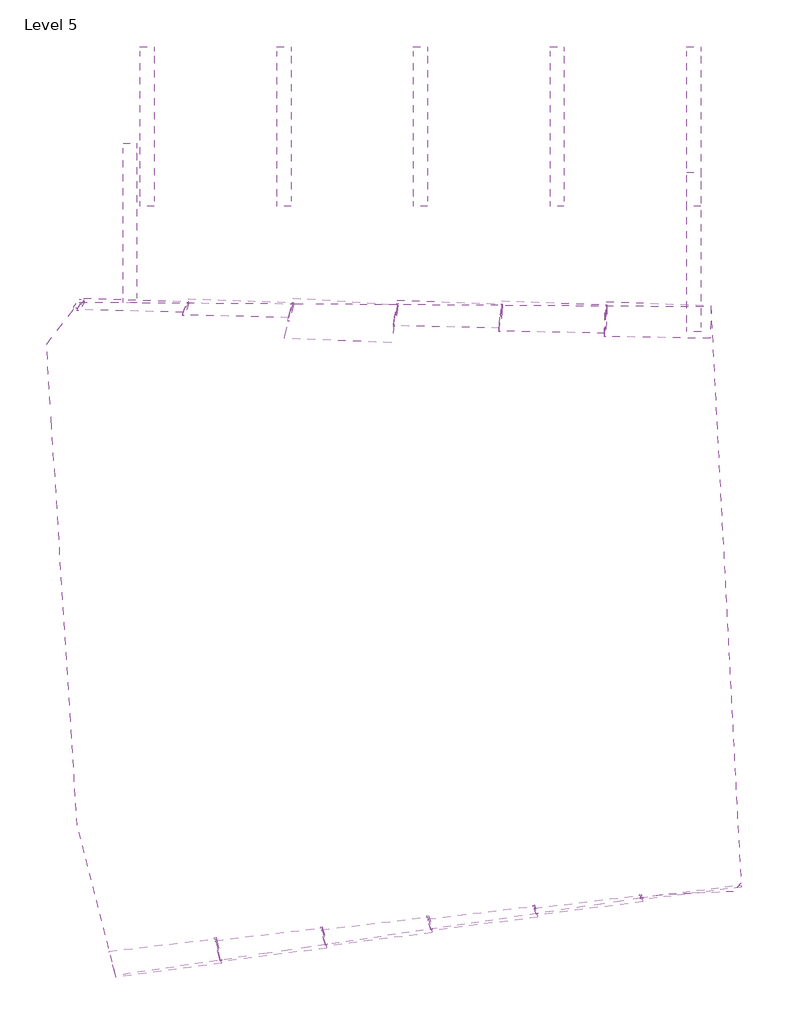
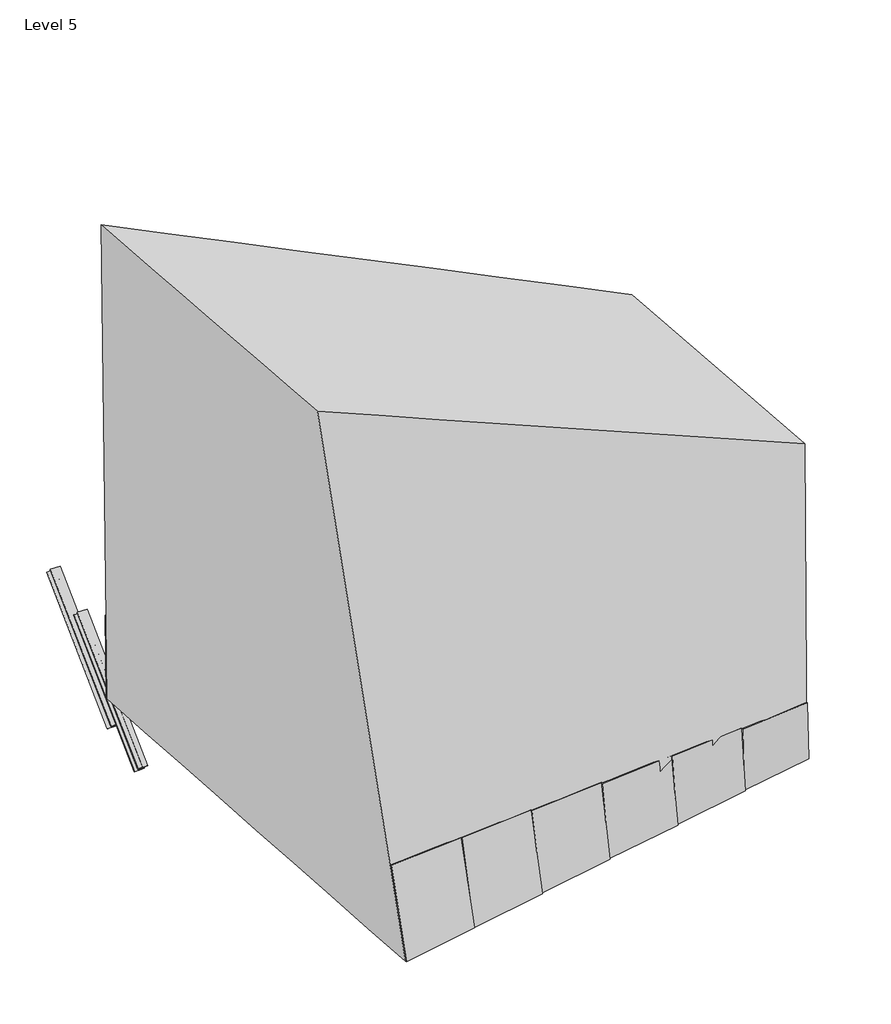
# One storey: 13 plates, 11 members, 7 columns, 1 proxy.
"""IFC4 building model written with IfcOpenShell, lengths in millimetres."""

import ifcopenshell
import ifcopenshell.guid

model = None  # the IFC model being written
_history = None  # IfcOwnerHistory: only IFC2X3 demands one
_inside = {}  # id of a spatial element -> (the spatial element, [elements in it])
_under = {}  # id of a project, library or spatial element -> (it, [spatial elements below it])
_declared = {}  # id of a project -> (the project, [libraries it declares])
_typed = {}  # id of a type object -> (the type object, [elements of that type])
_made_of = {}  # id of a material, layer set ... -> (it, [elements and type objects made of it])


def new_model(schema):
    """Start an empty IFC model of exactly this schema.

    Asked for "IFC4X3", IfcOpenShell would pick the latest addendum, in which some entities
    have other attributes; the version numbers below select the first issue.
    IFC2X3 requires an IfcOwnerHistory on every rooted entity: one is made here for all.
    """
    global model, _history
    if schema == "IFC4X3":
        model = ifcopenshell.file(schema_version=(4, 3, 0, 0))
    else:
        model = ifcopenshell.file(schema=schema)
    _inside.clear()
    _under.clear()
    _declared.clear()
    _typed.clear()
    _made_of.clear()
    _history = None
    if model.schema == "IFC2X3":
        org = make("IfcOrganization", Name="unknown")
        user = make(
            "IfcPersonAndOrganization",
            ThePerson=make("IfcPerson", FamilyName="unknown"),
            TheOrganization=org,
        )
        app = make(
            "IfcApplication",
            ApplicationDeveloper=org,
            Version="unknown",
            ApplicationFullName="unknown",
            ApplicationIdentifier="unknown",
        )
        _history = make(
            "IfcOwnerHistory",
            OwningUser=user,
            OwningApplication=app,
            ChangeAction="ADDED",
            CreationDate=0,
        )
    return model


def make(cls, **values):
    """One entity of the class cls with the attributes given. An attribute that is None is left unset."""
    return model.create_entity(
        cls, **{name: value for name, value in values.items() if value is not None}
    )


def rooted(cls, **values):
    """An entity with a GlobalId (a new one), such as an element, a storey or a relation."""
    return make(cls, GlobalId=ifcopenshell.guid.new(), OwnerHistory=_history, **values)


def si_unit(unit_type, name, prefix=None):
    """IfcSIUnit, for example si_unit("LENGTHUNIT", "METRE", prefix="MILLI")."""
    return make("IfcSIUnit", UnitType=unit_type, Prefix=prefix, Name=name)


def assignment(units):
    """IfcUnitAssignment: the units of a project."""
    return None if units is None else make("IfcUnitAssignment", Units=units)


def point(xyz):
    """IfcCartesianPoint."""
    return None if xyz is None else make("IfcCartesianPoint", Coordinates=xyz)


def direction(xyz):
    """IfcDirection."""
    return None if xyz is None else make("IfcDirection", DirectionRatios=xyz)


def frame(location, z_axis=None, x_axis=None):
    """IfcAxis2Placement3D, a coordinate frame: its origin and axes. An axis left out is left unset."""
    return make(
        "IfcAxis2Placement3D",
        Location=point(location),
        Axis=direction(z_axis),
        RefDirection=direction(x_axis),
    )


def frame_2d(location, x_axis=None):
    """IfcAxis2Placement2D, a coordinate frame in the plane: its origin and x axis."""
    return make(
        "IfcAxis2Placement2D", Location=point(location), RefDirection=direction(x_axis)
    )


def origin():
    """The frame at (0, 0, 0) with its axes left unset."""
    return frame((0.0, 0.0, 0.0))


def place(relative_to, where):
    """IfcLocalPlacement: puts the frame where relative to a parent placement (None: the world)."""
    return make(
        "IfcLocalPlacement", PlacementRelTo=relative_to, RelativePlacement=where
    )


def context(
    kind, dimensions, precision=None, world=None, true_north=None, identifier=None
):
    """IfcGeometricRepresentationContext, for example the 3D "Model" context."""
    return make(
        "IfcGeometricRepresentationContext",
        ContextIdentifier=identifier,
        ContextType=kind,
        CoordinateSpaceDimension=dimensions,
        Precision=precision,
        WorldCoordinateSystem=world,
        TrueNorth=true_north,
    )


def project(units=None, contexts=None):
    """IfcProject with its units and contexts."""
    return rooted(
        "IfcProject",
        Name="project",
        RepresentationContexts=contexts,
        UnitsInContext=assignment(units),
    )


def spatial(cls, under=None, at=None, **own):
    """A site, building, storey or space (cls), placed at a placement, below another one or the project."""
    s = rooted(cls, ObjectPlacement=at, **own)
    if under is not None:
        _under.setdefault(under.id(), (under, []))[1].append(s)
    return s


def polyline(points):
    """IfcPolyline through the points."""
    return make("IfcPolyline", Points=[point(p) for p in points])


def circle_curve(where, radius):
    """IfcCircle in the frame where."""
    return make("IfcCircle", Position=where, Radius=radius)


def trimmed(basis, trim1, trim2, sense, master):
    """IfcTrimmedCurve: the piece of a basis curve between two trims."""
    return make(
        "IfcTrimmedCurve",
        BasisCurve=basis,
        Trim1=trim1,
        Trim2=trim2,
        SenseAgreement=sense,
        MasterRepresentation=master,
    )


def segment(curve, same_sense, transition):
    """IfcCompositeCurveSegment."""
    return make(
        "IfcCompositeCurveSegment",
        Transition=transition,
        SameSense=same_sense,
        ParentCurve=curve,
    )


def composite_curve(segments, self_intersect=None):
    """IfcCompositeCurve: segments joined end to end."""
    return make("IfcCompositeCurve", Segments=segments, SelfIntersect=self_intersect)


def outline(outer, holes=None, kind="AREA"):
    """IfcArbitraryClosedProfileDef: a profile drawn as a closed curve; with holes, ...WithVoids."""
    if holes is None:
        return make("IfcArbitraryClosedProfileDef", ProfileType=kind, OuterCurve=outer)
    return make(
        "IfcArbitraryProfileDefWithVoids",
        ProfileType=kind,
        OuterCurve=outer,
        InnerCurves=holes,
    )


def extrude(swept, where, along, depth):
    """IfcExtrudedAreaSolid: the profile swept, set in the frame where, extruded along a direction by depth."""
    return make(
        "IfcExtrudedAreaSolid",
        SweptArea=swept,
        Position=where,
        ExtrudedDirection=direction(along),
        Depth=depth,
    )


def shape(context_of_items, identifier, shape_type, items):
    """IfcShapeRepresentation: the items that make up one representation, for example the "Body"."""
    return make(
        "IfcShapeRepresentation",
        ContextOfItems=context_of_items,
        RepresentationIdentifier=identifier,
        RepresentationType=shape_type,
        Items=items,
    )


def source(mapping_origin, context_of_items, identifier, shape_type, items):
    """IfcRepresentationMap: a shape defined once, which mapped items show again and again."""
    return make(
        "IfcRepresentationMap",
        MappingOrigin=mapping_origin,
        MappedRepresentation=shape(context_of_items, identifier, shape_type, items),
    )


def transform(
    local_origin,
    x_axis=None,
    y_axis=None,
    z_axis=None,
    scale=None,
    scale2=None,
    scale3=None,
    uniform=True,
):
    """IfcCartesianTransformationOperator3D, or its non-uniform kind. x_axis, y_axis, z_axis: its Axis1, 2, 3."""
    if uniform:
        return make(
            "IfcCartesianTransformationOperator3D",
            Axis1=direction(x_axis),
            Axis2=direction(y_axis),
            LocalOrigin=point(local_origin),
            Scale=scale,
            Axis3=direction(z_axis),
        )
    return make(
        "IfcCartesianTransformationOperator3DnonUniform",
        Axis1=direction(x_axis),
        Axis2=direction(y_axis),
        LocalOrigin=point(local_origin),
        Scale=scale,
        Axis3=direction(z_axis),
        Scale2=scale2,
        Scale3=scale3,
    )


def mapped(mapping_source, mapping_target):
    """IfcMappedItem: shows the shape of a source again, moved by a transform."""
    return make(
        "IfcMappedItem", MappingSource=mapping_source, MappingTarget=mapping_target
    )


def made_of(thing, what):
    """Note that an element or type object is made of a material, layer set ...; save() writes the relation."""
    if what is not None:
        _made_of.setdefault(what.id(), (what, []))[1].append(thing)
    return thing


def element(
    cls,
    number,
    at=None,
    inside=None,
    cuts=None,
    type_object=None,
    material=None,
    context=None,
    identifier="Body",
    shape_type=None,
    held_by="IfcProductDefinitionShape",
    body=None,
    shapes=None,
    **own,
):
    """One element of the class cls, such as IfcWall. Its Tag is "e" and its number.

    at: its placement. inside: the storey or other place that contains it. cuts: it is an
    opening in that element (IfcRelVoidsElement). A single representation is given by context,
    identifier, shape_type and body (its items); several are given by shapes. held_by: the class
    of the entity that holds the representations. save() writes the other relations.
    """
    e = rooted(cls, Tag="e%d" % number, ObjectPlacement=at, **own)
    if body is not None:
        shapes = [shape(context, identifier, shape_type, body)]
    if shapes is not None:
        e.Representation = make(held_by, Representations=shapes)
    if inside is not None:
        _inside.setdefault(inside.id(), (inside, []))[1].append(e)
    if cuts is not None:
        rooted(
            "IfcRelVoidsElement", RelatingBuildingElement=cuts, RelatedOpeningElement=e
        )
    if type_object is not None:
        _typed.setdefault(type_object.id(), (type_object, []))[1].append(e)
    return made_of(e, material)


def aggregate(whole, parts):
    """IfcRelAggregates: a whole, such as a stair, and the parts it consists of."""
    return rooted("IfcRelAggregates", RelatingObject=whole, RelatedObjects=parts)


def save(model, path):
    """Write the relations noted so far, then the file.

    IfcRelAggregates (storeys below a building ...), IfcRelContainedInSpatialStructure (elements
    in a storey), IfcRelDefinesByType, IfcRelAssociatesMaterial and IfcRelDeclares: one each for
    every whole, place, type object, material and project.
    """
    for whole, parts in _under.values():
        aggregate(whole, parts)
    for where, things in _inside.values():
        rooted(
            "IfcRelContainedInSpatialStructure",
            RelatedElements=things,
            RelatingStructure=where,
        )
    for kind, things in _typed.values():
        rooted("IfcRelDefinesByType", RelatedObjects=things, RelatingType=kind)
    for what, things in _made_of.values():
        rooted("IfcRelAssociatesMaterial", RelatedObjects=things, RelatingMaterial=what)
    for by, libraries in _declared.values():
        rooted("IfcRelDeclares", RelatingContext=by, RelatedDefinitions=libraries)
    model.write(path)


def spline_surface(u_degree, v_degree, points, u_multiplicities, v_multiplicities, u_knots, v_knots, weights=None):
    """IfcBSplineSurfaceWithKnots; with weights, IfcRationalBSplineSurfaceWithKnots. points: one row for each step in u."""
    own = dict(
        UDegree=u_degree,
        VDegree=v_degree,
        ControlPointsList=[[point(p) for p in row] for row in points],
        SurfaceForm="UNSPECIFIED",
        UClosed=False,
        VClosed=False,
        SelfIntersect=False,
        UMultiplicities=u_multiplicities,
        VMultiplicities=v_multiplicities,
        UKnots=u_knots,
        VKnots=v_knots,
        KnotSpec="UNSPECIFIED",
    )
    if weights is None:
        return make("IfcBSplineSurfaceWithKnots", **own)
    return make("IfcRationalBSplineSurfaceWithKnots", WeightsData=weights, **own)


def advanced_brep(points, edges, surfaces, faces):
    """IfcAdvancedBrep: a solid bounded by faces that lie on surfaces and meet in shared edges.

    An edge is (start, end): straight between two places in points (the first is 0);
    or (start, end, curve); or (start, end, curve, False) where it runs against its curve.
    A face is (place in surfaces, loops), or (place, loops, False) where it looks against
    its surface's normal. A loop lists edges by number (the first is 1), with a minus sign
    where the edge is run from its end to its start. The first loop is the outer one.
    """
    corners = [point(p) for p in points]
    vertices = [make("IfcVertexPoint", VertexGeometry=c) for c in corners]
    made = []
    for start, end, *more in edges:
        made.append(
            make(
                "IfcEdgeCurve",
                EdgeStart=vertices[start],
                EdgeEnd=vertices[end],
                EdgeGeometry=more[0] if more else make("IfcPolyline", Points=[corners[start], corners[end]]),
                SameSense=more[1] if len(more) > 1 else True,
            )
        )
    hull = []
    for where, loops, *sense in faces:
        bounds = []
        for j, loop in enumerate(loops):
            ring = [make("IfcOrientedEdge", EdgeElement=made[abs(k) - 1], Orientation=k > 0) for k in loop]
            bounds.append(
                make(
                    "IfcFaceOuterBound" if j == 0 else "IfcFaceBound",
                    Bound=make("IfcEdgeLoop", EdgeList=ring),
                    Orientation=True,
                )
            )
        hull.append(make("IfcAdvancedFace", Bounds=bounds, FaceSurface=surfaces[where], SameSense=sense[0] if sense else True))
    return make("IfcAdvancedBrep", Outer=make("IfcClosedShell", CfsFaces=hull))


def rectangular_mullion_30mm_square_281b7b6d(model_context):
    return source(origin(), model_context, "Body", "SweptSolid", [
        extrude(outline(polyline([(15.0, 15.0), (15.0, -15.0), (-15.0, -15.0), (-15.0, 15.0), (15.0, 15.0)])), frame((0.0, 0.0, -1763.4174675), z_axis=(0.0, 0.0, 1.0), x_axis=(1.0, 0.0, 0.0)), (0.0, 0.0, 1.0), 1763.4174675),
    ])


def rectangular_mullion_30mm_square_c8a39bf0(model_context):
    return source(origin(), model_context, "Body", "SweptSolid", [
        extrude(outline(polyline([(15.0, 15.0), (15.0, -15.0), (-15.0, -15.0), (-15.0, 15.0), (15.0, 15.0)])), frame((0.0, 0.0, -1876.7376356), z_axis=(0.0, 0.0, 1.0), x_axis=(1.0, 0.0, 0.0)), (0.0, 0.0, 1.0), 1876.7376356),
    ])


def rectangular_mullion_30mm_square_b082ce79(model_context):
    return source(origin(), model_context, "Body", "SweptSolid", [
        extrude(outline(polyline([(15.0, 15.0), (15.0, -15.0), (-15.0, -15.0), (-15.0, 15.0), (15.0, 15.0)])), frame((0.0, 0.0, -1997.4407133), z_axis=(0.0, 0.0, 1.0), x_axis=(1.0, 0.0, 0.0)), (0.0, 0.0, 1.0), 1997.4407133),
    ])


def rectangular_mullion_30mm_square_a1c2493b(model_context):
    return source(origin(), model_context, "Body", "SweptSolid", [
        extrude(outline(polyline([(15.0, 15.0), (15.0, -15.0), (-15.0, -15.0), (-15.0, 15.0), (15.0, 15.0)])), frame((0.0, 0.0, -2124.2685603), z_axis=(0.0, 0.0, 1.0), x_axis=(1.0, 0.0, 0.0)), (0.0, 0.0, 1.0), 2124.2685603),
    ])


def rectangular_mullion_30mm_square_b3fc8657(model_context):
    return source(origin(), model_context, "Body", "SweptSolid", [
        extrude(outline(polyline([(15.0, 15.0), (15.0, -15.0), (-15.0, -15.0), (-15.0, 15.0), (15.0, 15.0)])), frame((0.0, 0.0, -2256.188532), z_axis=(0.0, 0.0, 1.0), x_axis=(1.0, 0.0, 0.0)), (0.0, 0.0, 1.0), 2256.188532),
    ])


def rectangular_mullion_30mm_square_3a89077b(model_context):
    return source(origin(), model_context, "Body", "SweptSolid", [
        extrude(outline(polyline([(15.0, 15.0), (15.0, -15.0), (-15.0, -15.0), (-15.0, 15.0), (15.0, 15.0)])), frame((0.0, 0.0, -2392.3584034), z_axis=(0.0, 0.0, 1.0), x_axis=(1.0, 0.0, 0.0)), (0.0, 0.0, 1.0), 2392.3584034),
    ])


def rectangular_mullion_30mm_square_25ecd6b2(model_context):
    return source(origin(), model_context, "Body", "SweptSolid", [
        extrude(outline(polyline([(15.0, 15.0), (15.0, -15.0), (-15.0, -15.0), (-15.0, 15.0), (15.0, 15.0)])), frame((0.0, 0.0, -2311.5857878), z_axis=(0.0, 0.0, 1.0), x_axis=(1.0, 0.0, 0.0)), (0.0, 0.0, 1.0), 2311.5857878),
    ])


def rectangular_mullion_30mm_square_fecaf73a(model_context):
    return source(origin(), model_context, "Body", "SweptSolid", [
        extrude(outline(polyline([(15.0, 15.0), (15.0, -15.0), (-15.0, -15.0), (-15.0, 15.0), (15.0, 15.0)])), frame((0.0, 0.0, -2152.3545613), z_axis=(0.0, 0.0, 1.0), x_axis=(1.0, 0.0, 0.0)), (0.0, 0.0, 1.0), 2152.3545613),
    ])


def rectangular_mullion_30mm_square_a7719491(model_context):
    return source(origin(), model_context, "Body", "SweptSolid", [
        extrude(outline(polyline([(15.0, 15.0), (15.0, -15.0), (-15.0, -15.0), (-15.0, 15.0), (15.0, 15.0)])), frame((0.0, 0.0, -1995.0714456), z_axis=(0.0, 0.0, 1.0), x_axis=(1.0, 0.0, 0.0)), (0.0, 0.0, 1.0), 1995.0714456),
    ])


def rectangular_mullion_30mm_square_8e68c213(model_context):
    return source(origin(), model_context, "Body", "SweptSolid", [
        extrude(outline(polyline([(15.0, 15.0), (15.0, -15.0), (-15.0, -15.0), (-15.0, 15.0), (15.0, 15.0)])), frame((0.0, 0.0, -1840.2360175), z_axis=(0.0, 0.0, 1.0), x_axis=(1.0, 0.0, 0.0)), (0.0, 0.0, 1.0), 1840.2360175),
    ])


def rectangular_mullion_30mm_square_54935cf5(model_context):
    return source(origin(), model_context, "Body", "SweptSolid", [
        extrude(outline(polyline([(15.0, 15.0), (15.0, -15.0), (-15.0, -15.0), (-15.0, 15.0), (15.0, 15.0)])), frame((0.0, 0.0, -1688.5217616), z_axis=(0.0, 0.0, 1.0), x_axis=(1.0, 0.0, 0.0)), (0.0, 0.0, 1.0), 1688.5217616),
    ])


def system_panel_glazed_61bd3bb4(model_context):
    return source(origin(), model_context, "Body", "SweptSolid", [
        extrude(outline(polyline([(0.0, -918.1552821), (0.0, 996.0695243), (1761.0937074, 931.9438881), (1655.9323013, -996.0695243), (0.0, -918.1552821)])), frame((0.0, -49.5, 0.0), z_axis=(0.0, 1.0, 0.0), x_axis=(0.0, 0.0, 1.0)), (0.0, 0.0, 1.0), 25.0),
    ])


def system_panel_glazed_ae3b4f36(model_context):
    return source(origin(), model_context, "Body", "SweptSolid", [
        extrude(outline(polyline([(0.0, -923.1075404), (0.0, 991.2413385), (1874.9756018, 936.3989323), (1761.0780772, -991.2413385), (0.0, -923.1075404)])), frame((0.0, -49.5, 0.0), z_axis=(0.0, 1.0, 0.0), x_axis=(0.0, 0.0, 1.0)), (0.0, 0.0, 1.0), 25.0),
    ])


def system_panel_glazed_7d8b04ef(model_context):
    return source(origin(), model_context, "Body", "SweptSolid", [
        extrude(outline(polyline([(0.0, -937.8383573), (0.0, 976.8018413), (2255.477521, 949.9625368), (2123.3255208, -976.8018413), (0.0, -937.8383573)])), frame((0.0, -49.5, 0.0), z_axis=(0.0, 1.0, 0.0), x_axis=(0.0, 0.0, 1.0)), (0.0, 0.0, 1.0), 25.0),
    ])


def system_panel_glazed_3b9d15b0(model_context):
    return source(origin(), model_context, "Body", "SweptSolid", [
        extrude(outline(polyline([(0.0, -942.7108166), (0.0, 972.0020553), (2391.8329241, 954.5438482), (2255.5087034, -972.0020553), (0.0, -942.7108166)])), frame((0.0, -49.5, 0.0), z_axis=(0.0, 1.0, 0.0), x_axis=(0.0, 0.0, 1.0)), (0.0, 0.0, 1.0), 25.0),
    ])


def system_panel_glazed_4dd55457(model_context):
    return source(origin(), model_context, "Body", "SweptSolid", [
        extrude(outline(polyline([(0.0, -30.1852095), (0.0, 48.8417218), (2397.9897252, 30.6680018), (2392.2849165, -48.8417218), (0.0, -30.1852095)])), frame((0.0, -49.5, 0.0), z_axis=(0.0, 1.0, 0.0), x_axis=(0.0, 0.0, 1.0)), (0.0, 0.0, 1.0), 25.0),
    ])


def system_panel_glazed_c41e03b4(model_context):
    return source(origin(), model_context, "Body", "SweptSolid", [
        extrude(outline(polyline([(0.0, -1008.7560992), (0.0, 941.2557286), (2310.4175162, 1008.7560992), (2471.2238346, -938.6456704), (0.0, -1008.7560992)])), frame((0.0, -49.5, 0.0), z_axis=(0.0, 1.0, 0.0), x_axis=(0.0, 0.0, 1.0)), (0.0, 0.0, 1.0), 25.0),
    ])


def system_panel_glazed_15b89219(model_context):
    return source(origin(), model_context, "Body", "SweptSolid", [
        extrude(outline(polyline([(0.0, -1007.0351176), (0.0, 942.9445704), (2151.1749822, 1007.0351176), (2310.4173325, -940.4629834), (0.0, -1007.0351176)])), frame((0.0, -49.5, 0.0), z_axis=(0.0, 1.0, 0.0), x_axis=(0.0, 0.0, 1.0)), (0.0, 0.0, 1.0), 25.0),
    ])


def system_panel_glazed_cfa6e621(model_context):
    return source(origin(), model_context, "Body", "SweptSolid", [
        extrude(outline(polyline([(0.0, -1005.3178204), (0.0, 944.6224941), (1993.8665555, 1005.3178204), (2151.1709359, -942.2983527), (0.0, -1005.3178204)])), frame((0.0, -49.5, 0.0), z_axis=(0.0, 1.0, 0.0), x_axis=(0.0, 0.0, 1.0)), (0.0, 0.0, 1.0), 25.0),
    ])


def system_panel_glazed_fa6ac5bb(model_context):
    return source(origin(), model_context, "Body", "SweptSolid", [
        extrude(outline(polyline([(0.0, -1003.6052901), (0.0, 946.2862543), (1838.9863035, 1003.6052901), (1993.8564357, -944.1571371), (0.0, -1003.6052901)])), frame((0.0, -49.5, 0.0), z_axis=(0.0, 1.0, 0.0), x_axis=(0.0, 0.0, 1.0)), (0.0, 0.0, 1.0), 25.0),
    ])


def system_panel_glazed_53210cc6(model_context):
    return source(origin(), model_context, "Body", "SweptSolid", [
        extrude(outline(polyline([(0.0, -1001.8989904), (0.0, 947.931492), (1687.1996383, 1001.8989904), (1838.9666874, -946.0465604), (0.0, -1001.8989904)])), frame((0.0, -49.5, 0.0), z_axis=(0.0, 1.0, 0.0), x_axis=(0.0, 0.0, 1.0)), (0.0, 0.0, 1.0), 25.0),
    ])


def system_panel_glazed_08f6996d(model_context):
    return source(origin(), model_context, "Body", "SweptSolid", [
        extrude(outline(polyline([(0.0, -938.7563704), (0.0, 887.9536467), (1548.6739711, 938.7563704), (1687.2330704, -886.4668133), (0.0, -938.7563704)])), frame((0.0, -49.5, 0.0), z_axis=(0.0, 1.0, 0.0), x_axis=(0.0, 0.0, 1.0)), (0.0, 0.0, 1.0), 25.0),
    ])


def system_panel_glazed_6e61295c(model_context):
    return source(origin(), model_context, "Body", "SweptSolid", [
        extrude(outline(polyline([(0.0, -906.0305588), (0.0, 1006.3483292), (2123.3277595, 971.552521), (4246.6555191, 936.7567127), (3992.2264945, -1006.3483292), (1996.1132472, -956.189444), (0.0, -906.0305588)])), frame((0.0, -49.5, 0.0), z_axis=(0.0, 1.0, 0.0), x_axis=(0.0, 0.0, 1.0)), (0.0, 0.0, 1.0), 25.0),
    ])


def system_panel_glazed_31f0a782(model_context):
    return source(origin(), model_context, "Body", "SweptSolid", [
        extrude(outline(polyline([(0.0, -928.0385226), (0.0, 986.4208083), (1996.1252593, 940.8873527), (1874.9814945, -986.4208083), (0.0, -928.0385226)])), frame((0.0, -49.5, 0.0), z_axis=(0.0, 1.0, 0.0), x_axis=(0.0, 0.0, 1.0)), (0.0, 0.0, 1.0), 25.0),
    ])


model = new_model("IFC4")

# Units and contexts
model_context = context("Model", 3, world=origin())
ifc_project = project(units=[si_unit("LENGTHUNIT", "METRE", prefix="MILLI")], contexts=[model_context])

# Site, building, storey
site = spatial("IfcSite", under=ifc_project)
building = spatial("IfcBuilding", under=site)
storey = spatial("IfcBuildingStorey", under=building, Name="Level 5", Elevation=-5000.0)

# Proxy
placement = place(None, origin())
element("IfcBuildingElementProxy", 1, Name="volumen2 : volumen2", ObjectType="volumen2 : volumen2", at=placement, inside=storey, context=model_context, shape_type="AdvancedBrep", body=[
    advanced_brep(
    [(-4919.3716289, 29199.3093249, 0.0), (-5472.2265132, 39751.3413148, 0.0), (-5508.4633275, 36083.0409484, 8786.8733417), (-5062.165814, 29050.9821784, 8786.8733417), (-17027.8343957, 39830.0880172, -587.2378435), (-17626.1101206, 39059.1200592, 13141.9598572), (-16359.3479239, 27514.3891838, -587.2378435), (-17064.1810196, 30263.3944457, 13141.9598572)],
    [
        (0, 1),
        (1, 2),
        (2, 3),
        (3, 0),
        (1, 4),
        (4, 5),
        (5, 2),
        (4, 6),
        (6, 7),
        (7, 5),
        (6, 0),
        (3, 7),
    ],
    [
        spline_surface(1, 1, [[(-4919.3716289, 29199.3093249, 0.0), (-5062.165814, 29050.9821784, 8786.8733417)], [(-5472.2265132, 39751.3413148, 0.0), (-5508.4633275, 36083.0409484, 8786.8733417)]], [2, 2], [2, 2], [0.0, 1.0], [0.0, 1.0]),
        spline_surface(1, 1, [[(-5472.2265132, 39751.3413148, 0.0), (-5508.4633275, 36083.0409484, 8786.8733417)], [(-17027.8343957, 39830.0880172, -587.2378435), (-17626.1101206, 39059.1200592, 13141.9598572)]], [2, 2], [2, 2], [0.0, 1.0], [0.0, 1.0]),
        spline_surface(1, 1, [[(-17027.8343957, 39830.0880172, -587.2378435), (-17626.1101206, 39059.1200592, 13141.9598572)], [(-16359.3479239, 27514.3891838, -587.2378435), (-17064.1810196, 30263.3944457, 13141.9598572)]], [2, 2], [2, 2], [0.0, 1.0], [0.0, 1.0]),
        spline_surface(1, 1, [[(-16359.3479239, 27514.3891838, -587.2378435), (-17064.1810196, 30263.3944457, 13141.9598572)], [(-4919.3716289, 29199.3093249, 0.0), (-5062.165814, 29050.9821784, 8786.8733417)]], [2, 2], [2, 2], [0.0, 1.0], [0.0, 1.0]),
        spline_surface(1, 1, [[(-17064.1810196, 30263.3944457, 13141.9598572), (-17626.1101206, 39059.1200592, 13141.9598572)], [(-5062.165814, 29050.9821784, 8786.8733417), (-5508.4633275, 36083.0409484, 8786.8733417)]], [2, 2], [2, 2], [0.0, 1.0], [0.0, 1.0]),
        spline_surface(1, 1, [[(-16359.3479239, 27514.3891838, -587.2378435), (-4919.3716289, 29199.3093249, 0.0)], [(-17027.8343957, 39830.0880172, -587.2378435), (-5472.2265132, 39751.3413148, 0.0)]], [2, 2], [2, 2], [0.0, 1.0], [0.0, 1.0]),
    ],
    [
        (0, [[1, 2, 3, 4]]),
        (1, [[5, 6, 7, -2]]),
        (2, [[8, 9, 10, -6]]),
        (3, [[11, -4, 12, -9]]),
        (4, [[-10, -12, -3, -7]]),
        (5, [[-11, -8, -5, -1]]),
    ],
),
])

# Columns
element("IfcColumn", 2, ObjectType="M_W Shapes-Column : W250X73", at=placement, inside=storey, context=model_context, shape_type="SweptSolid", body=[
    extrude(outline(composite_curve([segment(polyline([(254.0, 0.0), (254.0, -14.2), (144.02, -14.2)]), True, "CONTINUOUS"), segment(trimmed(circle_curve(frame_2d((144.02, -26.9)), 12.7), [point((144.02, -14.2))], [point((131.32, -26.9))], True, "CARTESIAN"), True, "CONTINUOUS"), segment(polyline([(131.32, -26.9), (131.32, -227.1)]), True, "CONTINUOUS"), segment(trimmed(circle_curve(frame_2d((144.02, -227.1)), 12.7), [point((131.32, -227.1))], [point((144.02, -239.8))], True, "CARTESIAN"), True, "CONTINUOUS"), segment(polyline([(144.02, -239.8), (254.0, -239.8), (254.0, -254.0), (0.0, -254.0), (0.0, -239.8), (109.98, -239.8)]), True, "CONTINUOUS"), segment(trimmed(circle_curve(frame_2d((109.98, -227.1)), 12.7), [point((109.98, -239.8))], [point((122.68, -227.1))], True, "CARTESIAN"), True, "CONTINUOUS"), segment(polyline([(122.68, -227.1), (122.68, -26.9)]), True, "CONTINUOUS"), segment(trimmed(circle_curve(frame_2d((109.98, -26.9)), 12.7), [point((122.68, -26.9))], [point((109.98, -14.2))], True, "CARTESIAN"), True, "CONTINUOUS"), segment(polyline([(109.98, -14.2), (0.0, -14.2), (0.0, 0.0), (254.0, 0.0)]), True, "CONTINUOUS")], self_intersect=False)), frame((-5654.6382157, 41587.2616115, -2795.3553834), z_axis=(0.0, 0.7184819062976688, 0.6955456493450793), x_axis=(-1.0, 0.0, 0.0)), (0.0, 0.0, 1.0), 3813.3951187),
])
element("IfcColumn", 3, ObjectType="M_W Shapes-Column : W250X73", at=placement, inside=storey, context=model_context, shape_type="SweptSolid", body=[
    extrude(outline(composite_curve([segment(polyline([(254.0, 0.0), (254.0, -14.2), (144.02, -14.2)]), True, "CONTINUOUS"), segment(trimmed(circle_curve(frame_2d((144.02, -26.9)), 12.7), [point((144.02, -14.2))], [point((131.32, -26.9))], True, "CARTESIAN"), True, "CONTINUOUS"), segment(polyline([(131.32, -26.9), (131.32, -227.1)]), True, "CONTINUOUS"), segment(trimmed(circle_curve(frame_2d((144.02, -227.1)), 12.7), [point((131.32, -227.1))], [point((144.02, -239.8))], True, "CARTESIAN"), True, "CONTINUOUS"), segment(polyline([(144.02, -239.8), (254.0, -239.8), (254.0, -254.0), (0.0, -254.0), (0.0, -239.8), (109.98, -239.8)]), True, "CONTINUOUS"), segment(trimmed(circle_curve(frame_2d((109.98, -227.1)), 12.7), [point((109.98, -239.8))], [point((122.68, -227.1))], True, "CARTESIAN"), True, "CONTINUOUS"), segment(polyline([(122.68, -227.1), (122.68, -26.9)]), True, "CONTINUOUS"), segment(trimmed(circle_curve(frame_2d((109.98, -26.9)), 12.7), [point((122.68, -26.9))], [point((109.98, -14.2))], True, "CARTESIAN"), True, "CONTINUOUS"), segment(polyline([(109.98, -14.2), (0.0, -14.2), (0.0, 0.0), (254.0, 0.0)]), True, "CONTINUOUS")], self_intersect=False)), frame((-8154.6382157, 41587.2616115, -2795.3553834), z_axis=(0.0, 0.7184819062976688, 0.6955456493450793), x_axis=(-1.0, 0.0, 0.0)), (0.0, 0.0, 1.0), 3813.3951187),
])
element("IfcColumn", 4, ObjectType="M_W Shapes-Column : W250X73", at=placement, inside=storey, context=model_context, shape_type="SweptSolid", body=[
    extrude(outline(composite_curve([segment(polyline([(254.0, 0.0), (254.0, -14.2), (144.02, -14.2)]), True, "CONTINUOUS"), segment(trimmed(circle_curve(frame_2d((144.02, -26.9)), 12.7), [point((144.02, -14.2))], [point((131.32, -26.9))], True, "CARTESIAN"), True, "CONTINUOUS"), segment(polyline([(131.32, -26.9), (131.32, -227.1)]), True, "CONTINUOUS"), segment(trimmed(circle_curve(frame_2d((144.02, -227.1)), 12.7), [point((131.32, -227.1))], [point((144.02, -239.8))], True, "CARTESIAN"), True, "CONTINUOUS"), segment(polyline([(144.02, -239.8), (254.0, -239.8), (254.0, -254.0), (0.0, -254.0), (0.0, -239.8), (109.98, -239.8)]), True, "CONTINUOUS"), segment(trimmed(circle_curve(frame_2d((109.98, -227.1)), 12.7), [point((109.98, -239.8))], [point((122.68, -227.1))], True, "CARTESIAN"), True, "CONTINUOUS"), segment(polyline([(122.68, -227.1), (122.68, -26.9)]), True, "CONTINUOUS"), segment(trimmed(circle_curve(frame_2d((109.98, -26.9)), 12.7), [point((122.68, -26.9))], [point((109.98, -14.2))], True, "CARTESIAN"), True, "CONTINUOUS"), segment(polyline([(109.98, -14.2), (0.0, -14.2), (0.0, 0.0), (254.0, 0.0)]), True, "CONTINUOUS")], self_intersect=False)), frame((-10654.6382157, 41587.2616115, -2795.3553834), z_axis=(0.0, 0.7184819062976688, 0.6955456493450793), x_axis=(-1.0, 0.0, 0.0)), (0.0, 0.0, 1.0), 3813.3951187),
])
element("IfcColumn", 5, ObjectType="M_W Shapes-Column : W250X73", at=placement, inside=storey, context=model_context, shape_type="SweptSolid", body=[
    extrude(outline(composite_curve([segment(polyline([(254.0, 0.0), (254.0, -14.2), (144.02, -14.2)]), True, "CONTINUOUS"), segment(trimmed(circle_curve(frame_2d((144.02, -26.9)), 12.7), [point((144.02, -14.2))], [point((131.32, -26.9))], True, "CARTESIAN"), True, "CONTINUOUS"), segment(polyline([(131.32, -26.9), (131.32, -227.1)]), True, "CONTINUOUS"), segment(trimmed(circle_curve(frame_2d((144.02, -227.1)), 12.7), [point((131.32, -227.1))], [point((144.02, -239.8))], True, "CARTESIAN"), True, "CONTINUOUS"), segment(polyline([(144.02, -239.8), (254.0, -239.8), (254.0, -254.0), (0.0, -254.0), (0.0, -239.8), (109.98, -239.8)]), True, "CONTINUOUS"), segment(trimmed(circle_curve(frame_2d((109.98, -227.1)), 12.7), [point((109.98, -239.8))], [point((122.68, -227.1))], True, "CARTESIAN"), True, "CONTINUOUS"), segment(polyline([(122.68, -227.1), (122.68, -26.9)]), True, "CONTINUOUS"), segment(trimmed(circle_curve(frame_2d((109.98, -26.9)), 12.7), [point((122.68, -26.9))], [point((109.98, -14.2))], True, "CARTESIAN"), True, "CONTINUOUS"), segment(polyline([(109.98, -14.2), (0.0, -14.2), (0.0, 0.0), (254.0, 0.0)]), True, "CONTINUOUS")], self_intersect=False)), frame((-13154.6382157, 41587.2616115, -2795.3553834), z_axis=(0.0, 0.7184819062976688, 0.6955456493450793), x_axis=(-1.0, 0.0, 0.0)), (0.0, 0.0, 1.0), 3813.3951187),
])
element("IfcColumn", 6, ObjectType="M_W Shapes-Column : W250X73", at=placement, inside=storey, context=model_context, shape_type="SweptSolid", body=[
    extrude(outline(composite_curve([segment(polyline([(254.0, 0.0), (254.0, -14.2), (144.02, -14.2)]), True, "CONTINUOUS"), segment(trimmed(circle_curve(frame_2d((144.02, -26.9)), 12.7), [point((144.02, -14.2))], [point((131.32, -26.9))], True, "CARTESIAN"), True, "CONTINUOUS"), segment(polyline([(131.32, -26.9), (131.32, -227.1)]), True, "CONTINUOUS"), segment(trimmed(circle_curve(frame_2d((144.02, -227.1)), 12.7), [point((131.32, -227.1))], [point((144.02, -239.8))], True, "CARTESIAN"), True, "CONTINUOUS"), segment(polyline([(144.02, -239.8), (254.0, -239.8), (254.0, -254.0), (0.0, -254.0), (0.0, -239.8), (109.98, -239.8)]), True, "CONTINUOUS"), segment(trimmed(circle_curve(frame_2d((109.98, -227.1)), 12.7), [point((109.98, -239.8))], [point((122.68, -227.1))], True, "CARTESIAN"), True, "CONTINUOUS"), segment(polyline([(122.68, -227.1), (122.68, -26.9)]), True, "CONTINUOUS"), segment(trimmed(circle_curve(frame_2d((109.98, -26.9)), 12.7), [point((122.68, -26.9))], [point((109.98, -14.2))], True, "CARTESIAN"), True, "CONTINUOUS"), segment(polyline([(109.98, -14.2), (0.0, -14.2), (0.0, 0.0), (254.0, 0.0)]), True, "CONTINUOUS")], self_intersect=False)), frame((-15654.6382157, 41587.2616115, -2795.3553834), z_axis=(0.0, 0.7184819062976688, 0.6955456493450793), x_axis=(-1.0, 0.0, 0.0)), (0.0, 0.0, 1.0), 3813.3951187),
])
element("IfcColumn", 7, ObjectType="M_W Shapes-Column : W250X73", at=placement, inside=storey, context=model_context, shape_type="SweptSolid", body=[
    extrude(outline(composite_curve([segment(polyline([(254.0, 0.0), (254.0, -14.2), (144.02, -14.2)]), True, "CONTINUOUS"), segment(trimmed(circle_curve(frame_2d((144.02, -26.9)), 12.7), [point((144.02, -14.2))], [point((131.32, -26.9))], True, "CARTESIAN"), True, "CONTINUOUS"), segment(polyline([(131.32, -26.9), (131.32, -227.1)]), True, "CONTINUOUS"), segment(trimmed(circle_curve(frame_2d((144.02, -227.1)), 12.7), [point((131.32, -227.1))], [point((144.02, -239.8))], True, "CARTESIAN"), True, "CONTINUOUS"), segment(polyline([(144.02, -239.8), (254.0, -239.8), (254.0, -254.0), (0.0, -254.0), (0.0, -239.8), (109.98, -239.8)]), True, "CONTINUOUS"), segment(trimmed(circle_curve(frame_2d((109.98, -227.1)), 12.7), [point((109.98, -239.8))], [point((122.68, -227.1))], True, "CARTESIAN"), True, "CONTINUOUS"), segment(polyline([(122.68, -227.1), (122.68, -26.9)]), True, "CONTINUOUS"), segment(trimmed(circle_curve(frame_2d((109.98, -26.9)), 12.7), [point((122.68, -26.9))], [point((109.98, -14.2))], True, "CARTESIAN"), True, "CONTINUOUS"), segment(polyline([(109.98, -14.2), (0.0, -14.2), (0.0, 0.0), (254.0, 0.0)]), True, "CONTINUOUS")], self_intersect=False)), frame((-5654.6382157, 39287.2616115, -2795.3553834), z_axis=(0.0, 0.7184819062976688, 0.6955456493450793), x_axis=(-1.0, 0.0, 0.0)), (0.0, 0.0, 1.0), 3813.3951187),
])
element("IfcColumn", 8, ObjectType="M_W Shapes-Column : W250X73", at=placement, inside=storey, context=model_context, shape_type="SweptSolid", body=[
    extrude(outline(composite_curve([segment(polyline([(254.0, 0.0), (254.0, -14.2), (144.02, -14.2)]), True, "CONTINUOUS"), segment(trimmed(circle_curve(frame_2d((144.02, -26.9)), 12.7), [point((144.02, -14.2))], [point((131.32, -26.9))], True, "CARTESIAN"), True, "CONTINUOUS"), segment(polyline([(131.32, -26.9), (131.32, -227.1)]), True, "CONTINUOUS"), segment(trimmed(circle_curve(frame_2d((144.02, -227.1)), 12.7), [point((131.32, -227.1))], [point((144.02, -239.8))], True, "CARTESIAN"), True, "CONTINUOUS"), segment(polyline([(144.02, -239.8), (254.0, -239.8), (254.0, -254.0), (0.0, -254.0), (0.0, -239.8), (109.98, -239.8)]), True, "CONTINUOUS"), segment(trimmed(circle_curve(frame_2d((109.98, -227.1)), 12.7), [point((109.98, -239.8))], [point((122.68, -227.1))], True, "CARTESIAN"), True, "CONTINUOUS"), segment(polyline([(122.68, -227.1), (122.68, -26.9)]), True, "CONTINUOUS"), segment(trimmed(circle_curve(frame_2d((109.98, -26.9)), 12.7), [point((122.68, -26.9))], [point((109.98, -14.2))], True, "CARTESIAN"), True, "CONTINUOUS"), segment(polyline([(109.98, -14.2), (0.0, -14.2), (0.0, 0.0), (254.0, 0.0)]), True, "CONTINUOUS")], self_intersect=False)), frame((-15972.9054366, 39815.6255024, -2791.9681958), z_axis=(0.0, 0.7184819062976688, 0.6955456493450793), x_axis=(-1.0, 0.0, 0.0)), (0.0, 0.0, 1.0), 3813.3951187),
])

# Members
rectangular_mullion_30mm_square_shape = rectangular_mullion_30mm_square_281b7b6d(model_context)
element("IfcMember", 9, ObjectType="Rectangular Mullion : 30mm Square", at=placement, inside=storey, context=model_context, shape_type="MappedRepresentation", body=[
    mapped(rectangular_mullion_30mm_square_shape, transform((-7385.0035635, 39764.3761016, -97.2043255), x_axis=(-0.9998729452925407, -0.005028560353217801, -0.015126362840887234), y_axis=(-0.009537618578063182, 0.9490615348178275, 0.3149464033150544), z_axis=(0.012772122136885162, 0.3150506573711656, -0.9489889125728059))),
])
rectangular_mullion_30mm_square_2_shape = rectangular_mullion_30mm_square_c8a39bf0(model_context)
element("IfcMember", 10, ObjectType="Rectangular Mullion : 30mm Square", at=placement, inside=storey, context=model_context, shape_type="MappedRepresentation", body=[
    mapped(rectangular_mullion_30mm_square_2_shape, transform((-9297.7806022, 39777.4108883, -194.4086504), x_axis=(-0.9997679076944435, -0.00079270667948489, -0.02152910496038288), y_axis=(-0.006181711958080882, 0.9678558823700882, 0.2514294680400158), z_axis=(0.02063776105933496, 0.2515041999206739, -0.9676361507512623))),
])
rectangular_mullion_30mm_square_3_shape = rectangular_mullion_30mm_square_b082ce79(model_context)
element("IfcMember", 11, ObjectType="Rectangular Mullion : 30mm Square", at=placement, inside=storey, context=model_context, shape_type="MappedRepresentation", body=[
    mapped(rectangular_mullion_30mm_square_3_shape, transform((-11210.5576409, 39790.445675, -291.6129754), x_axis=(-0.9996165357843896, 0.0022133384670540712, -0.027602219462330026), y_axis=(-0.003197668495666148, 0.9809053073600256, 0.1944596433945251), z_axis=(0.027505568574530424, 0.19447333782748805, -0.9805220877530642))),
])
rectangular_mullion_30mm_square_4_shape = rectangular_mullion_30mm_square_a1c2493b(model_context)
element("IfcMember", 12, ObjectType="Rectangular Mullion : 30mm Square", at=placement, inside=storey, context=model_context, shape_type="MappedRepresentation", body=[
    mapped(rectangular_mullion_30mm_square_4_shape, transform((-13123.3346796, 39803.4804618, -388.8173003), x_axis=(-0.999438772340467, 0.004262373290087423, -0.03322608187127117), y_axis=(-0.000553024110512306, 0.9896371793517875, 0.14358951009377882), z_axis=(0.03349379803655682, 0.14352729851346802, -0.9890794103986353))),
])
rectangular_mullion_30mm_square_5_shape = rectangular_mullion_30mm_square_b3fc8657(model_context)
element("IfcMember", 13, ObjectType="Rectangular Mullion : 30mm Square", at=placement, inside=storey, context=model_context, shape_type="MappedRepresentation", body=[
    mapped(rectangular_mullion_30mm_square_5_shape, transform((-15036.1117183, 39816.5152485, -486.0216252), x_axis=(-0.9992485103462109, 0.005583022876058676, -0.03835680417401999), y_axis=(0.001789084109423265, 0.9951609015807584, 0.09824245081949805), z_axis=(0.03871968167389964, 0.0980999990853083, -0.994423036956875))),
])
rectangular_mullion_30mm_square_6_shape = rectangular_mullion_30mm_square_3a89077b(model_context)
element("IfcMember", 14, ObjectType="Rectangular Mullion : 30mm Square", at=placement, inside=storey, context=model_context, shape_type="MappedRepresentation", body=[
    mapped(rectangular_mullion_30mm_square_6_shape, transform((-16948.888757, 39829.5500352, -583.2259501), x_axis=(-0.9990550206425992, 0.006357944936474772, -0.04299584008948304), y_axis=(0.003865332846182831, 0.9983201276931695, 0.057809876705302785), z_axis=(0.04329116458128451, 0.057589054332215284, -0.9974013113538188))),
])
rectangular_mullion_30mm_square_7_shape = rectangular_mullion_30mm_square_25ecd6b2(model_context)
element("IfcMember", 15, ObjectType="Rectangular Mullion : 30mm Square", at=placement, inside=storey, context=model_context, shape_type="MappedRepresentation", body=[
    mapped(rectangular_mullion_30mm_square_7_shape, transform((-14432.4176202, 27798.1942893, -488.324492), x_axis=(0.9898208787839463, 0.14057908592015622, 0.022184420777417523), y_axis=(0.1344904984173129, -0.974927387709506, 0.17728196335042443), z_axis=(0.04655033575430946, -0.1724937949486062, -0.9839100349856126))),
])
rectangular_mullion_30mm_square_8_shape = rectangular_mullion_30mm_square_fecaf73a(model_context)
element("IfcMember", 16, ObjectType="Rectangular Mullion : 30mm Square", at=placement, inside=storey, context=model_context, shape_type="MappedRepresentation", body=[
    mapped(rectangular_mullion_30mm_square_8_shape, transform((-12505.487328, 28081.9993931, -389.4111411), x_axis=(0.9897335992450385, 0.14129415205815146, 0.02152591739345245), y_axis=(0.13654085783382, -0.9792512481434015, 0.1497450738808969), z_axis=(0.04223738471385663, -0.14526856371479233, -0.988490287119087))),
])
rectangular_mullion_30mm_square_9_shape = rectangular_mullion_30mm_square_a7719491(model_context)
element("IfcMember", 17, ObjectType="Rectangular Mullion : 30mm Square", at=placement, inside=storey, context=model_context, shape_type="MappedRepresentation", body=[
    mapped(rectangular_mullion_30mm_square_9_shape, transform((-10578.5570358, 28365.8044969, -290.4977903), x_axis=(0.9896239016020678, 0.14216640350428952, 0.020814588455132687), y_axis=(0.1387831819024312, -0.9833045234681792, 0.1176921515992195), z_axis=(0.037198948895603164, -0.11358225143776873, -0.9928319648154917))),
])
rectangular_mullion_30mm_square_10_shape = rectangular_mullion_30mm_square_8e68c213(model_context)
element("IfcMember", 18, ObjectType="Rectangular Mullion : 30mm Square", at=placement, inside=storey, context=model_context, shape_type="MappedRepresentation", body=[
    mapped(rectangular_mullion_30mm_square_10_shape, transform((-8651.6267436, 28649.6096007, -191.5844394), x_axis=(0.9894845134535597, 0.14324148801368472, 0.020056763128627645), y_axis=(0.14122121056007328, -0.9867367456384561, 0.08004476556762531), z_axis=(0.031256476505196626, -0.07637061554324454, -0.9965894650045355))),
])
rectangular_mullion_30mm_square_11_shape = rectangular_mullion_30mm_square_54935cf5(model_context)
element("IfcMember", 19, ObjectType="Rectangular Mullion : 30mm Square", at=placement, inside=storey, context=model_context, shape_type="MappedRepresentation", body=[
    mapped(rectangular_mullion_30mm_square_11_shape, transform((-6724.6964514, 28933.4147045, -92.6710885), x_axis=(0.9893054590337163, 0.1445799942949526, 0.01927002791278519), y_axis=(0.14384075630678256, -0.9889670287992309, 0.035412607544685955), z_axis=(0.024177376846565506, -0.032262070573548546, -0.9991869761216499))),
])

# Plates
system_panel_glazed_shape = system_panel_glazed_61bd3bb4(model_context)
element("IfcPlate", 20, ObjectType="System Panel : Glazed", at=placement, inside=storey, context=model_context, shape_type="MappedRepresentation", body=[
    mapped(system_panel_glazed_shape, transform((-6389.7159879, 39756.3760661, -47.0780472), x_axis=(-0.9985093709720135, 0.038058306394176226, -0.03912290116390964), y_axis=(-0.022011532229094022, -0.9367043961663445, -0.34942862883795284), z_axis=(-0.04994525533022723, -0.34804660538073234, 0.9361458390405564))),
])
system_panel_glazed_2_shape = system_panel_glazed_ae3b4f36(model_context)
element("IfcPlate", 21, ObjectType="System Panel : Glazed", at=placement, inside=storey, context=model_context, shape_type="MappedRepresentation", body=[
    mapped(system_panel_glazed_2_shape, transform((-8307.3783052, 39769.6372708, -144.3787485), x_axis=(-0.9984406747513097, 0.036875212281760106, -0.041909876178827375), y_axis=(-0.023544540996907524, -0.9588936425944761, -0.2827872641777604), z_axis=(-0.050614954226932324, -0.2813595580588522, 0.9582666254741072))),
])
system_panel_glazed_3_shape = system_panel_glazed_7d8b04ef(model_context)
element("IfcPlate", 22, ObjectType="System Panel : Glazed", at=placement, inside=storey, context=model_context, shape_type="MappedRepresentation", body=[
    mapped(system_panel_glazed_3_shape, transform((-14060.2739543, 39809.3616613, -436.4918796), x_axis=(-0.9983319085193589, 0.03265589948951582, -0.04761294635521912), y_axis=(-0.026679505118240812, -0.9922747965115182, -0.1211566432956572), z_axis=(-0.051201605821888985, -0.11968425308517405, 0.9914908346145738))),
])
system_panel_glazed_4_shape = system_panel_glazed_3b9d15b0(model_context)
element("IfcPlate", 23, ObjectType="System Panel : Glazed", at=placement, inside=storey, context=model_context, shape_type="MappedRepresentation", body=[
    mapped(system_panel_glazed_4_shape, transform((-15977.8792685, 39822.5746623, -533.9084684), x_axis=(-0.9983168898249081, 0.031270755549896924, -0.04884186050572829), y_axis=(-0.027378297540684826, -0.9965439344505364, -0.07842586010761356), z_axis=(-0.05112549573447834, -0.07695665375510964, 0.9957227812643036))),
])
system_panel_glazed_5_shape = system_panel_glazed_4dd55457(model_context)
element("IfcPlate", 24, ObjectType="System Panel : Glazed", at=placement, inside=storey, context=model_context, shape_type="MappedRepresentation", body=[
    mapped(system_panel_glazed_5_shape, transform((-16979.0490686, 39829.5338089, -584.7712305), x_axis=(-0.9983117521478105, 0.03057563294970559, -0.0493839669659436), y_axis=(-0.02769322004141189, -0.9979304987337345, -0.05803279470073622), z_axis=(-0.05105615621358969, -0.05656721989602046, 0.9970924824437946))),
])
system_panel_glazed_6_shape = system_panel_glazed_c41e03b4(model_context)
element("IfcPlate", 25, ObjectType="System Panel : Glazed", at=placement, inside=storey, context=model_context, shape_type="MappedRepresentation", body=[
    mapped(system_panel_glazed_6_shape, transform((-15362.472373, 27660.7137997, -535.9740692), x_axis=(0.989932312659797, 0.13102337262069855, 0.05354336727479423), y_axis=(-0.11877207297704269, 0.9747153016403859, -0.18927037652212675), z_axis=(-0.07698838245321156, 0.18100540482314104, 0.9804640903123627))),
])
system_panel_glazed_7_shape = system_panel_glazed_15b89219(model_context)
element("IfcPlate", 26, ObjectType="System Panel : Glazed", at=placement, inside=storey, context=model_context, shape_type="MappedRepresentation", body=[
    mapped(system_panel_glazed_7_shape, transform((-13437.2247747, 27944.2599212, -437.1586032), x_axis=(0.9900898297447399, 0.12991245083420452, 0.053337455453764504), y_axis=(-0.11967179792636372, 0.9792329043738972, -0.16365078604312747), z_axis=(-0.0734900661117099, 0.1556459897000636, 0.9850753961363486))),
])
system_panel_glazed_8_shape = system_panel_glazed_cfa6e621(model_context)
element("IfcPlate", 27, ObjectType="System Panel : Glazed", at=placement, inside=storey, context=model_context, shape_type="MappedRepresentation", body=[
    mapped(system_panel_glazed_8_shape, transform((-11511.9697486, 28227.8060652, -338.3451944), x_axis=(0.9902717449395044, 0.12864648619672217, 0.053027848944735806), y_axis=(-0.12060892990794786, 0.9836199026658261, -0.13396034154230366), z_axis=(-0.06939277484672932, 0.12626150905524414, 0.9895669124067173))),
])
system_panel_glazed_9_shape = system_panel_glazed_fa6ac5bb(model_context)
element("IfcPlate", 28, ObjectType="System Panel : Glazed", at=placement, inside=storey, context=model_context, shape_type="MappedRepresentation", body=[
    mapped(system_panel_glazed_9_shape, transform((-9586.7051259, 28511.3525292, -239.5344368), x_axis=(0.9904829494557039, 0.12719964261188088, 0.05257164403877235), y_axis=(-0.12156276512549655, 0.9876092683647103, -0.09924931826045577), z_axis=(-0.06454472071806473, 0.0919140030655376, 0.9936728813185433))),
])
system_panel_glazed_10_shape = system_panel_glazed_53210cc6(model_context)
element("IfcPlate", 29, ObjectType="System Panel : Glazed", at=placement, inside=storey, context=model_context, shape_type="MappedRepresentation", body=[
    mapped(system_panel_glazed_10_shape, transform((-7661.428011, 28794.8998222, -140.7271324), x_axis=(0.9907291343768793, 0.12554480923685474, 0.05190648486000074), y_axis=(-0.1224940455465101, 0.990755792076719, -0.05829381847231101), z_axis=(-0.05874513684118238, 0.05139514899399545, 0.9969491198438344))),
])
system_panel_glazed_11_shape = system_panel_glazed_08f6996d(model_context)
element("IfcPlate", 30, ObjectType="System Panel : Glazed", at=placement, inside=storey, context=model_context, shape_type="MappedRepresentation", body=[
    mapped(system_panel_glazed_11_shape, transform((-5796.86112, 29069.5047066, -45.0406455), x_axis=(0.9910067142020085, 0.12372139437500265, 0.0509775340757462), y_axis=(-0.12330760263306066, 0.9923053398449917, -0.0111958763838758), z_axis=(-0.051970448712956245, 0.004809271152771198, 0.9986370428596933))),
])
system_panel_glazed_12_shape = system_panel_glazed_6e61295c(model_context)
element("IfcPlate", 31, ObjectType="System Panel : Glazed", at=placement, inside=storey, context=model_context, shape_type="MappedRepresentation", body=[
    mapped(system_panel_glazed_12_shape, transform((-12116.9242956, 39793.8968209, -338.1354854), x_axis=(-0.9972682683355595, 0.061130694992198704, -0.04146129641925506), y_axis=(-0.05326444112323518, -0.9840517569223549, -0.16972047316059435), z_axis=(-0.05117519206435843, -0.1670484295879413, 0.9846196838827562))),
])
system_panel_glazed_13_shape = system_panel_glazed_31f0a782(model_context)
element("IfcPlate", 32, ObjectType="System Panel : Glazed", at=placement, inside=storey, context=model_context, shape_type="MappedRepresentation", body=[
    mapped(system_panel_glazed_13_shape, transform((-10225.0249555, 39782.8915616, -241.7202242), x_axis=(-0.9983907163064567, 0.035514886442372356, -0.04421165495732693), y_axis=(-0.02480167816314506, -0.9745536034357665, -0.2227782547526905), z_axis=(-0.05099857207189343, -0.22132321810272934, 0.9738660989968178))),
])

save(model, "model.ifc")

# Revit data of these elements
# Project information
#   Project Issue Date = "Issue Date"
#   Project Status = "Project  Status"
#   Client Name = "Maria Carrizo"
#   Project Address = "## Street\nCity, State  Zip"
#   Project Number = "Project  Number"
# Grids (mm)
#   "7": line (3552.58, 19337.645) -> (-12457.202, 19747.163)
#   "6": line (3641.067, 22796.966) -> (-13322.419, 22796.966)
#   "5": line (3717.805, 25796.966) -> (-13322.419, 25796.966)
#   "4": line (3641.067, 28953.259) -> (-10455.141, 29199.309)
#   "1": line (3717.805, 39899.667) -> (-21871.788, 39899.667)
#   "2": line (3717.805, 36899.667) -> (-21871.788, 36899.667)
#   "A": line (-17398.028, 47628.516) -> (-16178.976, 24760.987)
#   "B": line (-10138.967, 15594.116) -> (-12729.761, 42481.012)
#   "C": line (-6366.353, 15958.592) -> (-8928.85, 42551.825)
#   "D": line (-4918.869, 15958.592) -> (-4918.869, 29181.039)
#   "E": line (-2507.919, 16007.875) -> (-3787.774, 29290.03)
#   "F": line (1071.91, 16034.878) -> (-198.796, 29018.671)
#   "3": line (3717.805, 33899.667) -> (-21871.788, 33899.667)
# Type "M_W Shapes-Column : W250X73"
#   Section Name Key = "W10x49"
#   Width = 254 mm
#   Web Thickness = 8.64 mm
#   Web Fillet = 12.7 mm
#   Warping Constant = 556000 cm⁶
#   Torsional Moment of Inertia = 57.9 cm⁴
#   Section Area = 92.9 cm²
#   Plastic Modulus weak axis = 0.016386 (stored number, unit not read)
#   Plastic Modulus strong axis = 0.0349615 (stored number, unit not read)
#   Perimeter = 1.49 m²/m
#   Nominal Weight = 715.883 N/m
#   Moment of Inertia weak axis = 3890 cm⁴
#   Moment of Inertia strong axis = 11300 cm⁴
#   Height = 254 mm
#   Flange Thickness = 14.2 mm
#   Elastic Modulus weak axis = 0.0108063 (stored number, unit not read)
#   Elastic Modulus strong axis = 0.0316066 (stored number, unit not read)
#   Centroid Vertical = 127 mm
#   Centroid Horizontal = 127 mm
#   Structural Material [instance default] = Steel, 45-345
#   Assembly Code = ""
# Type "Rectangular Mullion : 30mm Square"
#   built-in parameter 1007304 = 0.0984252 (stored number, unit not read)
#   built-in parameter 1007301 = 0.0492126 (stored number, unit not read)
#   built-in parameter 1007300 = 0.0492126 (stored number, unit not read)
# Element 1 (IfcBuildingElementProxy, "volumen2 : volumen2")
#   Phase Created = New Construction
#   Materials on its faces: "Default Form"
# Elements 2, 3, 4, 5, 6, 7, 8 (IfcColumn, "M_W Shapes-Column : W250X73")
#   Comments = ""
#   Structural Material = Steel, 45-345
#   Phase Created = New Construction
#   Materials on its faces: "Steel, 45-345"
# Elements 9, 10, 11, 12, 13, 14, 15, 16, 17, 18, 19 (IfcMember, "Rectangular Mullion : 30mm Square")
#   Phase Created = New Construction
#   Materials on its faces: "Aluminum"
# Elements 20, 21, 22, 23, 24, 25, 26, 27, 28, 29, 30, 31, 32 (IfcPlate, "System Panel : Glazed")
#   Phase Created = New Construction
#   Materials on its faces: "Glass, Clear Glazing"
# Materials
#   "Steel, 45-345": class "Metal", colour RGB 189 187 185, transparency 0, Description = "Steel 345 MPa", Cost = 0
#   "Default Form": class "Generic", colour RGB 185 189 196, transparency 0.49, Cost = 0
#   "Aluminum": class "Metal", colour RGB 244 244 244, transparency 0, Description = "Aluminum 6061", Cost = 0
#   "Glass, Clear Glazing": class "Glass", colour RGB 247 249 248, transparency 0.85, Description = "Clear glazing", Cost = 0
